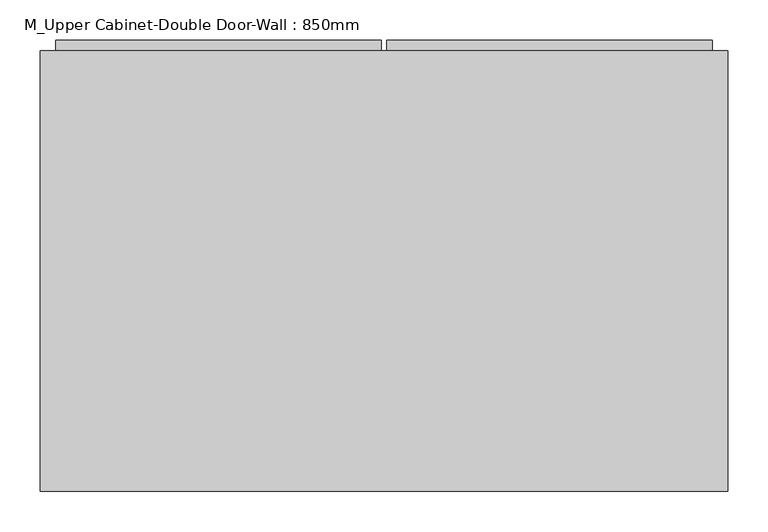
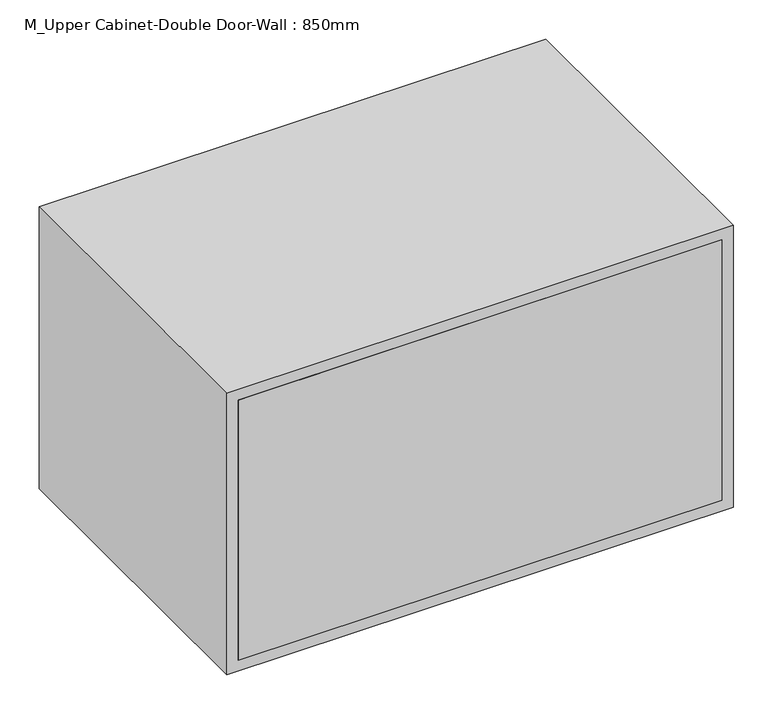
"""IFC4 building model written with IfcOpenShell, lengths in millimetres: furniture geometry, M_Upper Cabinet-Double Door-Wall : 850mm."""

from ifc_helpers import new_model, si_unit, frame, origin, place, context, project, spatial, polyline, outline, extrude, source, transform, mapped, element, save


def m_upper_cabinet_double_door_wall_850mm_b8bb223a(model_context):
    return source(origin(), model_context, "Body", "SweptSolid", [
        extrude(outline(polyline([(32.9461628, 645.2), (435.7211628, 645.2), (435.7211628, 613.45), (32.9461628, 613.45), (32.9461628, 645.2)])), frame((0.0, 0.0, 119.05), z_axis=(0.0, 0.0, 1.0), x_axis=(1.0, 0.0, 0.0)), (0.0, 0.0, 1.0), 461.9),
        extrude(outline(polyline([(-376.1788372, 645.2), (26.5961628, 645.2), (26.5961628, 613.45), (-376.1788372, 613.45), (-376.1788372, 645.2)])), frame((0.0, 0.0, 119.05), z_axis=(0.0, 0.0, 1.0), x_axis=(1.0, 0.0, 0.0)), (0.0, 0.0, 1.0), 461.9),
        extrude(outline(polyline([(435.7211628, 87.5), (-376.1788372, 87.5), (-376.1788372, 106.55), (435.7211628, 106.55), (435.7211628, 87.5)])), frame((0.0, 0.0, 119.05), z_axis=(0.0, 0.0, 1.0), x_axis=(1.0, 0.0, 0.0)), (0.0, 0.0, 1.0), 461.9),
        extrude(outline(polyline([(600.0, -395.2288372), (100.0, -395.2288372), (100.0, 454.7711628), (600.0, 454.7711628), (600.0, -395.2288372)]), holes=[polyline([(580.95, -376.1788372), (580.95, 435.7211628), (119.05, 435.7211628), (119.05, -376.1788372), (580.95, -376.1788372)])]), frame((0.0, 87.5, 0.0), z_axis=(0.0, 1.0, 0.0), x_axis=(0.0, 0.0, 1.0)), (0.0, 0.0, 1.0), 545.0),
    ])


if __name__ == "__main__":
    model = new_model("IFC4")
    model_context = context("Model", 3, world=origin())
    ifc_project = project(units=[si_unit("LENGTHUNIT", "METRE", prefix="MILLI")], contexts=[model_context])
    site = spatial("IfcSite", under=ifc_project)
    building = spatial("IfcBuilding", under=site)
    placement = place(None, origin())
    m_upper_cabinet_double_door_wall_850mm_shape = m_upper_cabinet_double_door_wall_850mm_b8bb223a(model_context)
    element("IfcFurniture", 1, ObjectType="M_Upper Cabinet-Double Door-Wall : 850mm", at=placement, inside=building, context=model_context, shape_type="MappedRepresentation", body=[
        mapped(m_upper_cabinet_double_door_wall_850mm_shape, transform((0.0, 0.0, 0.0), x_axis=(1.0, 0.0, 0.0), y_axis=(0.0, 1.0, 0.0), z_axis=(0.0, 0.0, 1.0))),
    ])
    save(model, "model.ifc")

# Revit data of these elements
# Type "M_Upper Cabinet-Double Door-Wall : 850mm"
#   COBie.Type.CreatedBy = "design@eagle.com"
#   COBie.Type.CreatedOn = "2016-09-01T06:50:21"
#   COBie.Type.Name = "Casework_M_Upper Cabinet-Double Door-Wall_850mm"
#   COBie.Type.Category = "23-40 35 17 47 11 : Kitchen Casework"
#   COBie.Type.Description = ""
#   COBie.Type.Manufacturer = ""
#   COBie.Type.ModelNumber = ""
#   COBie.Type.ReplacementCost = 0
#   Depth = 545 mm
#   Height = 500 mm
#   Top Of Cabinet = 600 mm
#   Width = 850 mm
#   COBie.Type = no
#   Cabinet Material = Door - Panel
#   Door/Drawer Material = Door - Panel
#   Handle Material = Cabinets - Handles
# Element 1 (IfcFurniture, "M_Upper Cabinet-Double Door-Wall : 850mm")
#   Materials on its faces: "Door - Panel"
# Materials
#   "Door - Panel": class "Wood", colour RGB 210 159 95, transparency 0
#   "Cabinets - Handles": class "Metal", colour RGB 57 57 57, transparency 0
